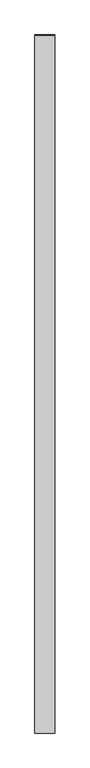
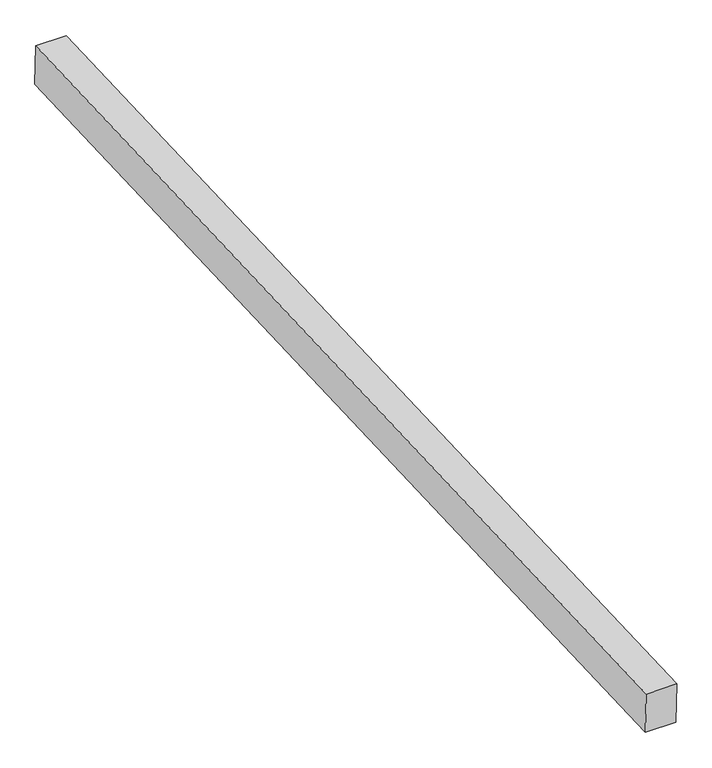
"""IFC4 building model written with IfcOpenShell, lengths in millimetres: proxy geometry, Generic Models 7:Generic Models 1:8:Generic Models 1:8 : Generic Models 7:Generic Models 1:337419:47 : Generic Models 7:Generic Models 1:8:Generic Models 1:8 : Generic Models 7:Generic Models 1:337419:315935."""

import ifcopenshell
import ifcopenshell.guid

model = None  # the IFC model being written
_history = None  # IfcOwnerHistory: only IFC2X3 demands one
_inside = {}  # id of a spatial element -> (the spatial element, [elements in it])
_under = {}  # id of a project, library or spatial element -> (it, [spatial elements below it])
_declared = {}  # id of a project -> (the project, [libraries it declares])
_typed = {}  # id of a type object -> (the type object, [elements of that type])
_made_of = {}  # id of a material, layer set ... -> (it, [elements and type objects made of it])


def new_model(schema):
    """Start an empty IFC model of exactly this schema.

    Asked for "IFC4X3", IfcOpenShell would pick the latest addendum, in which some entities
    have other attributes; the version numbers below select the first issue.
    IFC2X3 requires an IfcOwnerHistory on every rooted entity: one is made here for all.
    """
    global model, _history
    if schema == "IFC4X3":
        model = ifcopenshell.file(schema_version=(4, 3, 0, 0))
    else:
        model = ifcopenshell.file(schema=schema)
    _inside.clear()
    _under.clear()
    _declared.clear()
    _typed.clear()
    _made_of.clear()
    _history = None
    if model.schema == "IFC2X3":
        org = make("IfcOrganization", Name="unknown")
        user = make(
            "IfcPersonAndOrganization",
            ThePerson=make("IfcPerson", FamilyName="unknown"),
            TheOrganization=org,
        )
        app = make(
            "IfcApplication",
            ApplicationDeveloper=org,
            Version="unknown",
            ApplicationFullName="unknown",
            ApplicationIdentifier="unknown",
        )
        _history = make(
            "IfcOwnerHistory",
            OwningUser=user,
            OwningApplication=app,
            ChangeAction="ADDED",
            CreationDate=0,
        )
    return model


def make(cls, **values):
    """One entity of the class cls with the attributes given. An attribute that is None is left unset."""
    return model.create_entity(
        cls, **{name: value for name, value in values.items() if value is not None}
    )


def rooted(cls, **values):
    """An entity with a GlobalId (a new one), such as an element, a storey or a relation."""
    return make(cls, GlobalId=ifcopenshell.guid.new(), OwnerHistory=_history, **values)


def si_unit(unit_type, name, prefix=None):
    """IfcSIUnit, for example si_unit("LENGTHUNIT", "METRE", prefix="MILLI")."""
    return make("IfcSIUnit", UnitType=unit_type, Prefix=prefix, Name=name)


def assignment(units):
    """IfcUnitAssignment: the units of a project."""
    return None if units is None else make("IfcUnitAssignment", Units=units)


def point(xyz):
    """IfcCartesianPoint."""
    return None if xyz is None else make("IfcCartesianPoint", Coordinates=xyz)


def direction(xyz):
    """IfcDirection."""
    return None if xyz is None else make("IfcDirection", DirectionRatios=xyz)


def frame(location, z_axis=None, x_axis=None):
    """IfcAxis2Placement3D, a coordinate frame: its origin and axes. An axis left out is left unset."""
    return make(
        "IfcAxis2Placement3D",
        Location=point(location),
        Axis=direction(z_axis),
        RefDirection=direction(x_axis),
    )


def origin():
    """The frame at (0, 0, 0) with its axes left unset."""
    return frame((0.0, 0.0, 0.0))


def place(relative_to, where):
    """IfcLocalPlacement: puts the frame where relative to a parent placement (None: the world)."""
    return make(
        "IfcLocalPlacement", PlacementRelTo=relative_to, RelativePlacement=where
    )


def context(
    kind, dimensions, precision=None, world=None, true_north=None, identifier=None
):
    """IfcGeometricRepresentationContext, for example the 3D "Model" context."""
    return make(
        "IfcGeometricRepresentationContext",
        ContextIdentifier=identifier,
        ContextType=kind,
        CoordinateSpaceDimension=dimensions,
        Precision=precision,
        WorldCoordinateSystem=world,
        TrueNorth=true_north,
    )


def project(units=None, contexts=None):
    """IfcProject with its units and contexts."""
    return rooted(
        "IfcProject",
        Name="project",
        RepresentationContexts=contexts,
        UnitsInContext=assignment(units),
    )


def spatial(cls, under=None, at=None, **own):
    """A site, building, storey or space (cls), placed at a placement, below another one or the project."""
    s = rooted(cls, ObjectPlacement=at, **own)
    if under is not None:
        _under.setdefault(under.id(), (under, []))[1].append(s)
    return s


def polyline(points):
    """IfcPolyline through the points."""
    return make("IfcPolyline", Points=[point(p) for p in points])


def outline(outer, holes=None, kind="AREA"):
    """IfcArbitraryClosedProfileDef: a profile drawn as a closed curve; with holes, ...WithVoids."""
    if holes is None:
        return make("IfcArbitraryClosedProfileDef", ProfileType=kind, OuterCurve=outer)
    return make(
        "IfcArbitraryProfileDefWithVoids",
        ProfileType=kind,
        OuterCurve=outer,
        InnerCurves=holes,
    )


def extrude(swept, where, along, depth):
    """IfcExtrudedAreaSolid: the profile swept, set in the frame where, extruded along a direction by depth."""
    return make(
        "IfcExtrudedAreaSolid",
        SweptArea=swept,
        Position=where,
        ExtrudedDirection=direction(along),
        Depth=depth,
    )


def shape(context_of_items, identifier, shape_type, items):
    """IfcShapeRepresentation: the items that make up one representation, for example the "Body"."""
    return make(
        "IfcShapeRepresentation",
        ContextOfItems=context_of_items,
        RepresentationIdentifier=identifier,
        RepresentationType=shape_type,
        Items=items,
    )


def source(mapping_origin, context_of_items, identifier, shape_type, items):
    """IfcRepresentationMap: a shape defined once, which mapped items show again and again."""
    return make(
        "IfcRepresentationMap",
        MappingOrigin=mapping_origin,
        MappedRepresentation=shape(context_of_items, identifier, shape_type, items),
    )


def transform(
    local_origin,
    x_axis=None,
    y_axis=None,
    z_axis=None,
    scale=None,
    scale2=None,
    scale3=None,
    uniform=True,
):
    """IfcCartesianTransformationOperator3D, or its non-uniform kind. x_axis, y_axis, z_axis: its Axis1, 2, 3."""
    if uniform:
        return make(
            "IfcCartesianTransformationOperator3D",
            Axis1=direction(x_axis),
            Axis2=direction(y_axis),
            LocalOrigin=point(local_origin),
            Scale=scale,
            Axis3=direction(z_axis),
        )
    return make(
        "IfcCartesianTransformationOperator3DnonUniform",
        Axis1=direction(x_axis),
        Axis2=direction(y_axis),
        LocalOrigin=point(local_origin),
        Scale=scale,
        Axis3=direction(z_axis),
        Scale2=scale2,
        Scale3=scale3,
    )


def mapped(mapping_source, mapping_target):
    """IfcMappedItem: shows the shape of a source again, moved by a transform."""
    return make(
        "IfcMappedItem", MappingSource=mapping_source, MappingTarget=mapping_target
    )


def made_of(thing, what):
    """Note that an element or type object is made of a material, layer set ...; save() writes the relation."""
    if what is not None:
        _made_of.setdefault(what.id(), (what, []))[1].append(thing)
    return thing


def element(
    cls,
    number,
    at=None,
    inside=None,
    cuts=None,
    type_object=None,
    material=None,
    context=None,
    identifier="Body",
    shape_type=None,
    held_by="IfcProductDefinitionShape",
    body=None,
    shapes=None,
    **own,
):
    """One element of the class cls, such as IfcWall. Its Tag is "e" and its number.

    at: its placement. inside: the storey or other place that contains it. cuts: it is an
    opening in that element (IfcRelVoidsElement). A single representation is given by context,
    identifier, shape_type and body (its items); several are given by shapes. held_by: the class
    of the entity that holds the representations. save() writes the other relations.
    """
    e = rooted(cls, Tag="e%d" % number, ObjectPlacement=at, **own)
    if body is not None:
        shapes = [shape(context, identifier, shape_type, body)]
    if shapes is not None:
        e.Representation = make(held_by, Representations=shapes)
    if inside is not None:
        _inside.setdefault(inside.id(), (inside, []))[1].append(e)
    if cuts is not None:
        rooted(
            "IfcRelVoidsElement", RelatingBuildingElement=cuts, RelatedOpeningElement=e
        )
    if type_object is not None:
        _typed.setdefault(type_object.id(), (type_object, []))[1].append(e)
    return made_of(e, material)


def aggregate(whole, parts):
    """IfcRelAggregates: a whole, such as a stair, and the parts it consists of."""
    return rooted("IfcRelAggregates", RelatingObject=whole, RelatedObjects=parts)


def save(model, path):
    """Write the relations noted so far, then the file.

    IfcRelAggregates (storeys below a building ...), IfcRelContainedInSpatialStructure (elements
    in a storey), IfcRelDefinesByType, IfcRelAssociatesMaterial and IfcRelDeclares: one each for
    every whole, place, type object, material and project.
    """
    for whole, parts in _under.values():
        aggregate(whole, parts)
    for where, things in _inside.values():
        rooted(
            "IfcRelContainedInSpatialStructure",
            RelatedElements=things,
            RelatingStructure=where,
        )
    for kind, things in _typed.values():
        rooted("IfcRelDefinesByType", RelatedObjects=things, RelatingType=kind)
    for what, things in _made_of.values():
        rooted("IfcRelAssociatesMaterial", RelatedObjects=things, RelatingMaterial=what)
    for by, libraries in _declared.values():
        rooted("IfcRelDeclares", RelatingContext=by, RelatedDefinitions=libraries)
    model.write(path)


def generic_models_37406ff3(model_context):
    return source(origin(), model_context, "Body", "SweptSolid", [
        extrude(outline(polyline([(-581229.2495411, 3818.908703), (-576356.3266468, 4021.9471569), (-576348.7597251, 3831.5971524), (-581221.3189223, 3628.5738526), (-581229.2495411, 3818.908703)])), frame((613273.861724, 0.0, 0.0), z_axis=(1.0, 0.0, 0.0), x_axis=(0.0, 1.0, 0.0)), (0.0, 0.0, 1.0), 139.7),
    ])


if __name__ == "__main__":
    model = new_model("IFC4")
    model_context = context("Model", 3, world=origin())
    ifc_project = project(units=[si_unit("LENGTHUNIT", "METRE", prefix="MILLI")], contexts=[model_context])
    site = spatial("IfcSite", under=ifc_project)
    building = spatial("IfcBuilding", under=site)
    placement = place(None, origin())
    generic_models_shape = generic_models_37406ff3(model_context)
    element("IfcBuildingElementProxy", 1, Name="Generic Models 7:Generic Models 1:8:Generic Models 1:8 : Generic Models 7:Generic Models 1:337419:47 : Generic Models 7:Generic Models 1:8:Generic Models 1:8 : Generic Models 7:Generic Models 1:337419:315935", ObjectType="Generic Models 7:Generic Models 1:8:Generic Models 1:8 : Generic Models 7:Generic Models 1:337419:47 : Generic Models 7:Generic Models 1:8:Generic Models 1:8 : Generic Models 7:Generic Models 1:337419:315935", at=placement, inside=building, context=model_context, shape_type="MappedRepresentation", body=[
        mapped(generic_models_shape, transform((0.0, 0.0, 0.0), x_axis=(1.0, 0.0, 0.0), y_axis=(0.0, 1.0, 0.0), z_axis=(0.0, 0.0, 1.0))),
    ])
    save(model, "model.ifc")

# Revit data of these elements
# Type "Generic Models 7:Generic Models 1:8:Generic Models 1:8 : Generic Models 7:Generic Models 1:337419:47 : Generic Models 7:Generic Models 1:8:Generic Models 1:8 : Generic Models 7:Generic Models 1:337419:315935"
#   NameOverride = "Generic Models 7:Generic Models 1:8:Generic Models 1:8 : Generic Models 7:Generic Models 1:337419:315935"
#   ObjectTypeOverride = "Generic Models 1:8 : Generic Models 7:Generic Models 1:337419"
#   Reference = "Generic Models 1"
#   Tag = "315935"
# Element 1 (IfcBuildingElementProxy, "Generic Models 7:Generic Models 1:8:Generic Models 1:8 : Generic Models 7:Generic Models 1:337419:47 : Generic Models 7:Generic Models 1:8:Generic Models 1:8 : Generic Models 7:Generic Models 1:337419:315935")
#   Materials on its faces: "5 1/2\" X 7 1/2\" EXTERIOR GRADE GLULAM BEAMS"
# Materials
#   "5 1/2\" X 7 1/2\" EXTERIOR GRADE GLULAM BEAMS": class "Wood", colour RGB 183 134 68, transparency 0, Keynote = "M06181300.01", Description = "Pinus Echinata", Cost = 0
